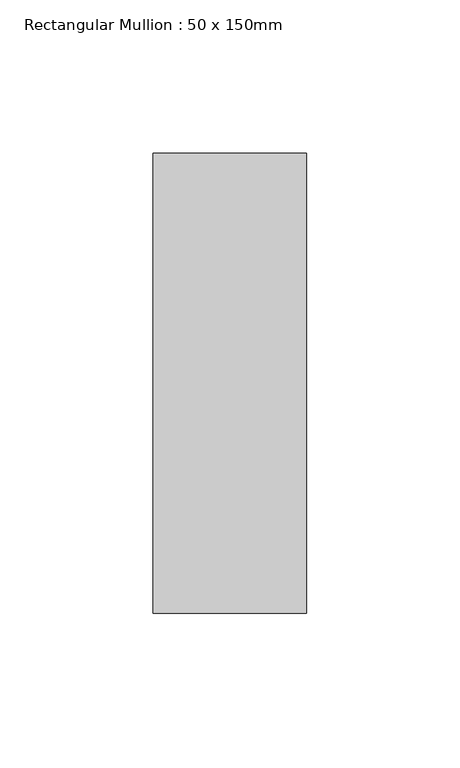
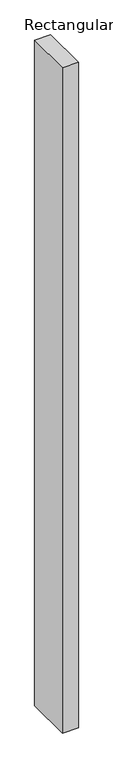
"""IFC4 building model written with IfcOpenShell, lengths in millimetres: member geometry, Rectangular Mullion : 50 x 150mm."""

from ifc_helpers import new_model, si_unit, frame, origin, place, context, project, spatial, polyline, outline, extrude, source, transform, mapped, element, save


def rectangular_mullion_50_x_150mm_792551fd(model_context):
    return source(origin(), model_context, "Body", "SweptSolid", [
        extrude(outline(polyline([(0.0, 75.0), (0.0, -75.0), (-50.0, -75.0), (-50.0, 75.0), (0.0, 75.0)])), frame((0.0, 0.0, -2200.0), z_axis=(0.0, 0.0, 1.0), x_axis=(1.0, 0.0, 0.0)), (0.0, 0.0, 1.0), 2200.0),
    ])


if __name__ == "__main__":
    model = new_model("IFC4")
    model_context = context("Model", 3, world=origin())
    ifc_project = project(units=[si_unit("LENGTHUNIT", "METRE", prefix="MILLI")], contexts=[model_context])
    site = spatial("IfcSite", under=ifc_project)
    building = spatial("IfcBuilding", under=site)
    placement = place(None, origin())
    rectangular_mullion_50_x_150mm_shape = rectangular_mullion_50_x_150mm_792551fd(model_context)
    element("IfcMember", 1, ObjectType="Rectangular Mullion : 50 x 150mm", at=placement, inside=building, context=model_context, shape_type="MappedRepresentation", body=[
        mapped(rectangular_mullion_50_x_150mm_shape, transform((0.0, 0.0, 0.0), x_axis=(1.0, 0.0, 0.0), y_axis=(0.0, 1.0, 0.0), z_axis=(0.0, 0.0, 1.0))),
    ])
    save(model, "model.ifc")

# Revit data of these elements
# Type "Rectangular Mullion : 50 x 150mm"
#   Keynote = "H11"
#   built-in parameter 1007304 = 0.492126 (stored number, unit not read)
#   built-in parameter 1007301 = 0.082021 (stored number, unit not read)
#   built-in parameter 1007300 = 0.082021 (stored number, unit not read)
# Element 1 (IfcMember, "Rectangular Mullion : 50 x 150mm")
#   Materials on its faces: "Aluminium"
# Materials
#   "Aluminium": class "Metal", colour RGB 247 247 247, transparency 0, Description = "Aluminium 6061", Cost = 0
